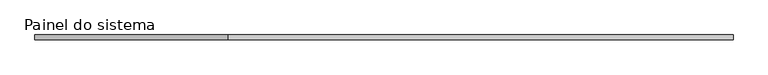
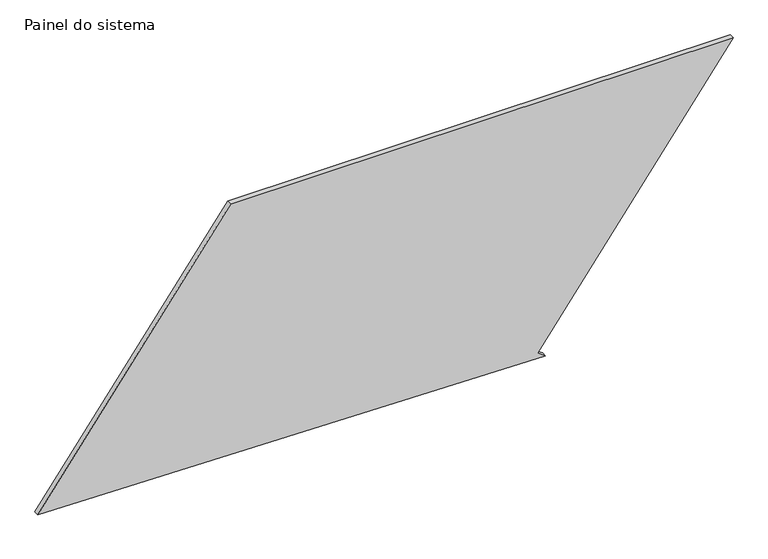
"""IFC4 building model written with IfcOpenShell, lengths in millimetres: plate geometry, Painel do sistema : Envidraçado."""

from ifc_helpers import new_model, si_unit, frame, origin, place, context, project, spatial, polyline, outline, extrude, source, transform, mapped, element, save


def painel_do_sistema_159b9050(model_context):
    return source(origin(), model_context, "Body", "SweptSolid", [
        extrude(outline(polyline([(0.0, 815.5008223), (29.674901, 775.2590498), (1381.6710836, 1772.2417958), (1381.6710836, -789.5927946), (49.112718, -1772.2417958), (0.0, 815.5008223)])), frame((0.0, 24.5, 0.0), z_axis=(0.0, 1.0, 0.0), x_axis=(0.0, 0.0, 1.0)), (0.0, 0.0, 1.0), 25.0),
    ])


if __name__ == "__main__":
    model = new_model("IFC4")
    model_context = context("Model", 3, world=origin())
    ifc_project = project(units=[si_unit("LENGTHUNIT", "METRE", prefix="MILLI")], contexts=[model_context])
    site = spatial("IfcSite", under=ifc_project)
    building = spatial("IfcBuilding", under=site)
    placement = place(None, origin())
    painel_do_sistema_shape = painel_do_sistema_159b9050(model_context)
    element("IfcPlate", 1, ObjectType="Painel do sistema : Envidraçado", at=placement, inside=building, context=model_context, shape_type="MappedRepresentation", body=[
        mapped(painel_do_sistema_shape, transform((0.0, 0.0, 0.0), x_axis=(1.0, 0.0, 0.0), y_axis=(0.0, 1.0, 0.0), z_axis=(0.0, 0.0, 1.0))),
    ])
    save(model, "model.ifc")

# Revit data of these elements
# Type "Painel do sistema : Envidraçado"
#   Construction Type Id = "GSP4R"
#   Analytic Construction = "Vidraça única Pilkington 1/8 pol"
#   Visual Light Transmittance = 0.9
#   Solar Heat Gain Coefficient = 0.86
#   Heat Transfer Coefficient (U) = 6.7069 W/(m²·K)
# Element 1 (IfcPlate, "Painel do sistema : Envidraçado")
#   Materials on its faces: "Vidro"
# Materials
#   "Vidro": class "Vidro", colour RGB 0 128 192, transparency 0.9, Description = "Vidro de sílica", Cost = 0
